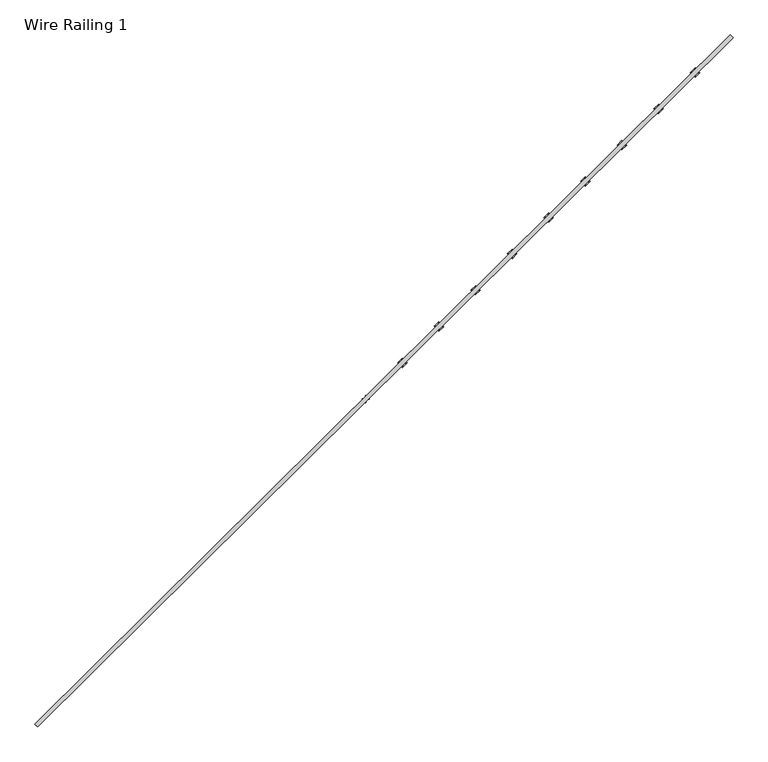
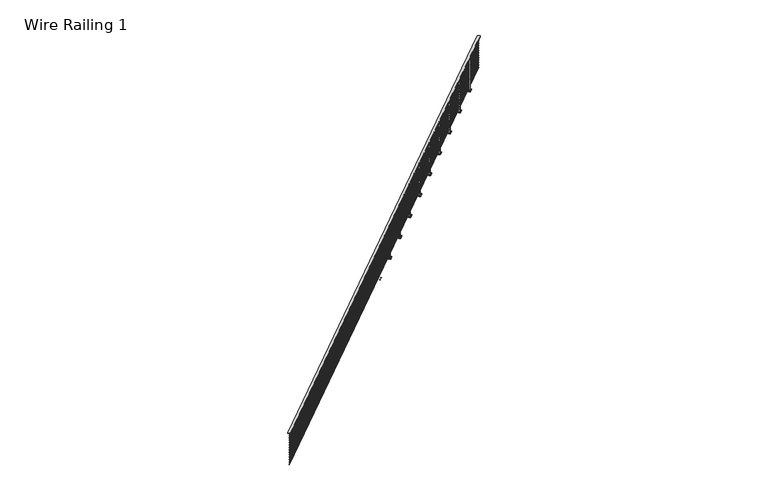
"""IFC4 building model written with IfcOpenShell, lengths in millimetres: railing geometry, Wire Railing 1."""

from ifc_helpers import new_model, si_unit, point, frame, frame_2d, origin, place, context, project, spatial, polyline, circle_curve, trimmed, segment, composite_curve, outline, extrude, source, transform, mapped, element, save


def wire_railing_1_765eeab6(model_context):
    return source(origin(), model_context, "Body", "SweptSolid", [
        extrude(outline(polyline([(32583.8298074, 24310.825617), (32530.1909697, 24364.9487644), (45743.1001377, 37459.6249857), (45796.7389755, 37405.5018383), (32583.8298074, 24310.825617)])), frame((0.0, 0.0, 265004.55), z_axis=(0.0, 0.0, 1.0), x_axis=(1.0, 0.0, 0.0)), (0.0, 0.0, 1.0), 19.05),
        extrude(outline(composite_curve([segment(trimmed(circle_curve(frame_2d((0.0, 2.38125)), 2.38125), [point((-2.38125, 2.38125))], [point((2.38125, 2.38125))], False, "CARTESIAN"), True, "CONTINUOUS"), segment(trimmed(circle_curve(frame_2d((0.0, 2.38125)), 2.38125), [point((2.38125, 2.38125))], [point((-2.38125, 2.38125))], False, "CARTESIAN"), True, "CONTINUOUS")], self_intersect=False)), frame((32557.0103886, 24337.8871907, 264947.4), z_axis=(0.7102775248505508, 0.7039217553763878, 0.0), x_axis=(0.7039217553763878, -0.7102775248505508, 0.0)), (0.0, 0.0, 1.0), 18602.4598918),
        extrude(outline(composite_curve([segment(trimmed(circle_curve(frame_2d((0.0, 2.38125)), 2.38125), [point((-2.38125, 2.38125))], [point((2.38125, 2.38125))], False, "CARTESIAN"), True, "CONTINUOUS"), segment(trimmed(circle_curve(frame_2d((0.0, 2.38125)), 2.38125), [point((2.38125, 2.38125))], [point((-2.38125, 2.38125))], False, "CARTESIAN"), True, "CONTINUOUS")], self_intersect=False)), frame((32557.0103886, 24337.8871907, 264871.2), z_axis=(0.7102775248505508, 0.7039217553763878, 0.0), x_axis=(0.7039217553763878, -0.7102775248505508, 0.0)), (0.0, 0.0, 1.0), 18602.4598918),
        extrude(outline(composite_curve([segment(trimmed(circle_curve(frame_2d((0.0, 2.38125)), 2.38125), [point((-2.38125, 2.38125))], [point((2.38125, 2.38125))], False, "CARTESIAN"), True, "CONTINUOUS"), segment(trimmed(circle_curve(frame_2d((0.0, 2.38125)), 2.38125), [point((2.38125, 2.38125))], [point((-2.38125, 2.38125))], False, "CARTESIAN"), True, "CONTINUOUS")], self_intersect=False)), frame((32557.0103886, 24337.8871907, 264795.0), z_axis=(0.7102775248505508, 0.7039217553763878, 0.0), x_axis=(0.7039217553763878, -0.7102775248505508, 0.0)), (0.0, 0.0, 1.0), 18602.4598918),
        extrude(outline(composite_curve([segment(trimmed(circle_curve(frame_2d((0.0, 2.38125)), 2.38125), [point((-2.38125, 2.38125))], [point((2.38125, 2.38125))], False, "CARTESIAN"), True, "CONTINUOUS"), segment(trimmed(circle_curve(frame_2d((0.0, 2.38125)), 2.38125), [point((2.38125, 2.38125))], [point((-2.38125, 2.38125))], False, "CARTESIAN"), True, "CONTINUOUS")], self_intersect=False)), frame((32557.0103886, 24337.8871907, 264718.8), z_axis=(0.7102775248505508, 0.7039217553763878, 0.0), x_axis=(0.7039217553763878, -0.7102775248505508, 0.0)), (0.0, 0.0, 1.0), 18602.4598918),
        extrude(outline(composite_curve([segment(trimmed(circle_curve(frame_2d((0.0, 2.38125)), 2.38125), [point((-2.38125, 2.38125))], [point((2.38125, 2.38125))], False, "CARTESIAN"), True, "CONTINUOUS"), segment(trimmed(circle_curve(frame_2d((0.0, 2.38125)), 2.38125), [point((2.38125, 2.38125))], [point((-2.38125, 2.38125))], False, "CARTESIAN"), True, "CONTINUOUS")], self_intersect=False)), frame((32557.0103886, 24337.8871907, 264642.6), z_axis=(0.7102775248505508, 0.7039217553763878, 0.0), x_axis=(0.7039217553763878, -0.7102775248505508, 0.0)), (0.0, 0.0, 1.0), 18602.4598918),
        extrude(outline(composite_curve([segment(trimmed(circle_curve(frame_2d((0.0, 2.38125)), 2.38125), [point((-2.38125, 2.38125))], [point((2.38125, 2.38125))], False, "CARTESIAN"), True, "CONTINUOUS"), segment(trimmed(circle_curve(frame_2d((0.0, 2.38125)), 2.38125), [point((2.38125, 2.38125))], [point((-2.38125, 2.38125))], False, "CARTESIAN"), True, "CONTINUOUS")], self_intersect=False)), frame((32557.0103886, 24337.8871907, 264566.4), z_axis=(0.7102775248505508, 0.7039217553763878, 0.0), x_axis=(0.7039217553763878, -0.7102775248505508, 0.0)), (0.0, 0.0, 1.0), 18602.4598918),
        extrude(outline(composite_curve([segment(trimmed(circle_curve(frame_2d((0.0, 2.38125)), 2.38125), [point((-2.38125, 2.38125))], [point((2.38125, 2.38125))], False, "CARTESIAN"), True, "CONTINUOUS"), segment(trimmed(circle_curve(frame_2d((0.0, 2.38125)), 2.38125), [point((2.38125, 2.38125))], [point((-2.38125, 2.38125))], False, "CARTESIAN"), True, "CONTINUOUS")], self_intersect=False)), frame((32557.0103886, 24337.8871907, 264490.2), z_axis=(0.7102775248505508, 0.7039217553763878, 0.0), x_axis=(0.7039217553763878, -0.7102775248505508, 0.0)), (0.0, 0.0, 1.0), 18602.4598918),
        extrude(outline(composite_curve([segment(trimmed(circle_curve(frame_2d((0.0, 2.38125)), 2.38125), [point((-2.38125, 2.38125))], [point((2.38125, 2.38125))], False, "CARTESIAN"), True, "CONTINUOUS"), segment(trimmed(circle_curve(frame_2d((0.0, 2.38125)), 2.38125), [point((2.38125, 2.38125))], [point((-2.38125, 2.38125))], False, "CARTESIAN"), True, "CONTINUOUS")], self_intersect=False)), frame((32557.0103886, 24337.8871907, 264414.0), z_axis=(0.7102775248505508, 0.7039217553763878, 0.0), x_axis=(0.7039217553763878, -0.7102775248505508, 0.0)), (0.0, 0.0, 1.0), 18602.4598918),
        extrude(outline(composite_curve([segment(trimmed(circle_curve(frame_2d((0.0, 2.38125)), 2.38125), [point((-2.38125, 2.38125))], [point((2.38125, 2.38125))], False, "CARTESIAN"), True, "CONTINUOUS"), segment(trimmed(circle_curve(frame_2d((0.0, 2.38125)), 2.38125), [point((2.38125, 2.38125))], [point((-2.38125, 2.38125))], False, "CARTESIAN"), True, "CONTINUOUS")], self_intersect=False)), frame((32557.0103886, 24337.8871907, 264337.8), z_axis=(0.7102775248505508, 0.7039217553763878, 0.0), x_axis=(0.7039217553763878, -0.7102775248505508, 0.0)), (0.0, 0.0, 1.0), 18602.4598918),
        extrude(outline(composite_curve([segment(trimmed(circle_curve(frame_2d((0.0, 2.38125)), 2.38125), [point((-2.38125, 2.38125))], [point((2.38125, 2.38125))], False, "CARTESIAN"), True, "CONTINUOUS"), segment(trimmed(circle_curve(frame_2d((0.0, 2.38125)), 2.38125), [point((2.38125, 2.38125))], [point((-2.38125, 2.38125))], False, "CARTESIAN"), True, "CONTINUOUS")], self_intersect=False)), frame((32557.0103886, 24337.8871907, 264261.6), z_axis=(0.7102775248505508, 0.7039217553763878, 0.0), x_axis=(0.7039217553763878, -0.7102775248505508, 0.0)), (0.0, 0.0, 1.0), 18602.4598918),
        extrude(outline(composite_curve([segment(trimmed(circle_curve(frame_2d((0.0, 2.38125)), 2.38125), [point((-2.38125, 2.38125))], [point((2.38125, 2.38125))], False, "CARTESIAN"), True, "CONTINUOUS"), segment(trimmed(circle_curve(frame_2d((0.0, 2.38125)), 2.38125), [point((2.38125, 2.38125))], [point((-2.38125, 2.38125))], False, "CARTESIAN"), True, "CONTINUOUS")], self_intersect=False)), frame((32557.0103886, 24337.8871907, 264185.4), z_axis=(0.7102775248505508, 0.7039217553763878, 0.0), x_axis=(0.7039217553763878, -0.7102775248505508, 0.0)), (0.0, 0.0, 1.0), 18602.4598918),
        extrude(outline(composite_curve([segment(trimmed(circle_curve(frame_2d((0.0, 2.38125)), 2.38125), [point((-2.38125, 2.38125))], [point((2.38125, 2.38125))], False, "CARTESIAN"), True, "CONTINUOUS"), segment(trimmed(circle_curve(frame_2d((0.0, 2.38125)), 2.38125), [point((2.38125, 2.38125))], [point((-2.38125, 2.38125))], False, "CARTESIAN"), True, "CONTINUOUS")], self_intersect=False)), frame((32557.0103886, 24337.8871907, 264109.2), z_axis=(0.7102775248505508, 0.7039217553763878, 0.0), x_axis=(0.7039217553763878, -0.7102775248505508, 0.0)), (0.0, 0.0, 1.0), 18602.4598918),
        extrude(outline(composite_curve([segment(trimmed(circle_curve(frame_2d((0.0, 2.38125)), 2.38125), [point((-2.38125, 2.38125))], [point((2.38125, 2.38125))], False, "CARTESIAN"), True, "CONTINUOUS"), segment(trimmed(circle_curve(frame_2d((0.0, 2.38125)), 2.38125), [point((2.38125, 2.38125))], [point((-2.38125, 2.38125))], False, "CARTESIAN"), True, "CONTINUOUS")], self_intersect=False)), frame((32557.0103886, 24337.8871907, 264033.0), z_axis=(0.7102775248505508, 0.7039217553763878, 0.0), x_axis=(0.7039217553763878, -0.7102775248505508, 0.0)), (0.0, 0.0, 1.0), 18602.4598918),
        extrude(outline(composite_curve([segment(trimmed(circle_curve(frame_2d((45074.2207706, 36680.5087687)), 6.35), [point((45078.6906738, 36675.9985064))], [point((45069.7508675, 36685.019031))], False, "CARTESIAN"), True, "CONTINUOUS"), segment(trimmed(circle_curve(frame_2d((45074.2207706, 36680.5087687)), 6.35), [point((45069.7508675, 36685.019031))], [point((45078.6906738, 36675.9985064))], False, "CARTESIAN"), True, "CONTINUOUS")], self_intersect=False)), frame((0.0, 0.0, 263956.8), z_axis=(0.0, 0.0, 1.0), x_axis=(1.0, 0.0, 0.0)), (0.0, 0.0, 1.0), 12.7),
        extrude(outline(composite_curve([segment(trimmed(circle_curve(frame_2d((45011.6421266, 36743.6524406)), 6.35), [point((45016.1120297, 36739.1421784))], [point((45007.1722234, 36748.1627029))], False, "CARTESIAN"), True, "CONTINUOUS"), segment(trimmed(circle_curve(frame_2d((45011.6421266, 36743.6524406)), 6.35), [point((45007.1722234, 36748.1627029))], [point((45016.1120297, 36739.1421784))], False, "CARTESIAN"), True, "CONTINUOUS")], self_intersect=False)), frame((0.0, 0.0, 263956.8), z_axis=(0.0, 0.0, 1.0), x_axis=(1.0, 0.0, 0.0)), (0.0, 0.0, 1.0), 12.7),
        extrude(outline(composite_curve([segment(trimmed(circle_curve(frame_2d((45137.3644426, 36743.0874127)), 6.35), [point((45141.8343458, 36738.5771505))], [point((45132.8945395, 36747.597675))], False, "CARTESIAN"), True, "CONTINUOUS"), segment(trimmed(circle_curve(frame_2d((45137.3644426, 36743.0874127)), 6.35), [point((45132.8945395, 36747.597675))], [point((45141.8343458, 36738.5771505))], False, "CARTESIAN"), True, "CONTINUOUS")], self_intersect=False)), frame((0.0, 0.0, 263956.8), z_axis=(0.0, 0.0, 1.0), x_axis=(1.0, 0.0, 0.0)), (0.0, 0.0, 1.0), 12.7),
        extrude(outline(composite_curve([segment(trimmed(circle_curve(frame_2d((45074.7857986, 36806.2310847)), 6.35), [point((45079.2557017, 36801.7208224))], [point((45070.3158954, 36810.741347))], False, "CARTESIAN"), True, "CONTINUOUS"), segment(trimmed(circle_curve(frame_2d((45074.7857986, 36806.2310847)), 6.35), [point((45070.3158954, 36810.741347))], [point((45079.2557017, 36801.7208224))], False, "CARTESIAN"), True, "CONTINUOUS")], self_intersect=False)), frame((0.0, 0.0, 263956.8), z_axis=(0.0, 0.0, 1.0), x_axis=(1.0, 0.0, 0.0)), (0.0, 0.0, 1.0), 12.7),
        extrude(outline(polyline([(44984.7016303, 36743.7735181), (45074.906876, 36833.171581), (45164.3049389, 36742.9663353), (45074.0996932, 36653.5682724), (44984.7016303, 36743.7735181)])), frame((0.0, 0.0, 263956.8), z_axis=(0.0, 0.0, 1.0), x_axis=(1.0, 0.0, 0.0)), (0.0, 0.0, 1.0), 6.35),
        extrude(outline(polyline([(45031.8474988, 36743.5616326), (45074.6949905, 36786.0257125), (45117.1590704, 36743.1782208), (45074.3115787, 36700.7141409), (45031.8474988, 36743.5616326)]), holes=[polyline([(45040.8276642, 36743.5212735), (45074.3519378, 36709.6943063), (45108.178905, 36743.2185799), (45074.6546314, 36777.0455471), (45040.8276642, 36743.5212735)])]), frame((0.0, 0.0, 263956.8), z_axis=(0.0, 0.0, 1.0), x_axis=(1.0, 0.0, 0.0)), (0.0, 0.0, 1.0), 1047.75),
        extrude(outline(composite_curve([segment(trimmed(circle_curve(frame_2d((44378.8044986, 35991.3152834)), 6.35), [point((44383.2744018, 35986.8050211))], [point((44374.3345955, 35995.8255456))], False, "CARTESIAN"), True, "CONTINUOUS"), segment(trimmed(circle_curve(frame_2d((44378.8044986, 35991.3152834)), 6.35), [point((44374.3345955, 35995.8255456))], [point((44383.2744018, 35986.8050211))], False, "CARTESIAN"), True, "CONTINUOUS")], self_intersect=False)), frame((0.0, 0.0, 263956.8), z_axis=(0.0, 0.0, 1.0), x_axis=(1.0, 0.0, 0.0)), (0.0, 0.0, 1.0), 12.7),
        extrude(outline(composite_curve([segment(trimmed(circle_curve(frame_2d((44316.2258546, 36054.4589553)), 6.35), [point((44320.6957577, 36049.948693))], [point((44311.7559514, 36058.9692176))], False, "CARTESIAN"), True, "CONTINUOUS"), segment(trimmed(circle_curve(frame_2d((44316.2258546, 36054.4589553)), 6.35), [point((44311.7559514, 36058.9692176))], [point((44320.6957577, 36049.948693))], False, "CARTESIAN"), True, "CONTINUOUS")], self_intersect=False)), frame((0.0, 0.0, 263956.8), z_axis=(0.0, 0.0, 1.0), x_axis=(1.0, 0.0, 0.0)), (0.0, 0.0, 1.0), 12.7),
        extrude(outline(composite_curve([segment(trimmed(circle_curve(frame_2d((44441.9481706, 36053.8939274)), 6.35), [point((44446.4180738, 36049.3836651))], [point((44437.4782675, 36058.4041897))], False, "CARTESIAN"), True, "CONTINUOUS"), segment(trimmed(circle_curve(frame_2d((44441.9481706, 36053.8939274)), 6.35), [point((44437.4782675, 36058.4041897))], [point((44446.4180738, 36049.3836651))], False, "CARTESIAN"), True, "CONTINUOUS")], self_intersect=False)), frame((0.0, 0.0, 263956.8), z_axis=(0.0, 0.0, 1.0), x_axis=(1.0, 0.0, 0.0)), (0.0, 0.0, 1.0), 12.7),
        extrude(outline(composite_curve([segment(trimmed(circle_curve(frame_2d((44379.3695266, 36117.0375994)), 6.35), [point((44383.8394297, 36112.5273371))], [point((44374.8996234, 36121.5478616))], False, "CARTESIAN"), True, "CONTINUOUS"), segment(trimmed(circle_curve(frame_2d((44379.3695266, 36117.0375994)), 6.35), [point((44374.8996234, 36121.5478616))], [point((44383.8394297, 36112.5273371))], False, "CARTESIAN"), True, "CONTINUOUS")], self_intersect=False)), frame((0.0, 0.0, 263956.8), z_axis=(0.0, 0.0, 1.0), x_axis=(1.0, 0.0, 0.0)), (0.0, 0.0, 1.0), 12.7),
        extrude(outline(polyline([(44289.2853583, 36054.5800327), (44379.490604, 36143.9780957), (44468.8886669, 36053.77285), (44378.6834212, 35964.3747871), (44289.2853583, 36054.5800327)])), frame((0.0, 0.0, 263956.8), z_axis=(0.0, 0.0, 1.0), x_axis=(1.0, 0.0, 0.0)), (0.0, 0.0, 1.0), 6.35),
        extrude(outline(polyline([(44336.4312268, 36054.3681473), (44379.2787185, 36096.8322271), (44421.7427984, 36053.9847355), (44378.8953067, 36011.5206556), (44336.4312268, 36054.3681473)]), holes=[polyline([(44345.4113922, 36054.3277881), (44378.9356658, 36020.500821), (44412.762633, 36054.0250946), (44379.2383594, 36087.8520617), (44345.4113922, 36054.3277881)])]), frame((0.0, 0.0, 263956.8), z_axis=(0.0, 0.0, 1.0), x_axis=(1.0, 0.0, 0.0)), (0.0, 0.0, 1.0), 1047.75),
        extrude(outline(composite_curve([segment(trimmed(circle_curve(frame_2d((43683.3882266, 35302.121798)), 6.35), [point((43687.8581298, 35297.6115357))], [point((43678.9183235, 35306.6320603))], False, "CARTESIAN"), True, "CONTINUOUS"), segment(trimmed(circle_curve(frame_2d((43683.3882266, 35302.121798)), 6.35), [point((43678.9183235, 35306.6320603))], [point((43687.8581298, 35297.6115357))], False, "CARTESIAN"), True, "CONTINUOUS")], self_intersect=False)), frame((0.0, 0.0, 263956.8), z_axis=(0.0, 0.0, 1.0), x_axis=(1.0, 0.0, 0.0)), (0.0, 0.0, 1.0), 12.7),
        extrude(outline(composite_curve([segment(trimmed(circle_curve(frame_2d((43620.8095826, 35365.26547)), 6.35), [point((43625.2794857, 35360.7552077))], [point((43616.3396794, 35369.7757323))], False, "CARTESIAN"), True, "CONTINUOUS"), segment(trimmed(circle_curve(frame_2d((43620.8095826, 35365.26547)), 6.35), [point((43616.3396794, 35369.7757323))], [point((43625.2794857, 35360.7552077))], False, "CARTESIAN"), True, "CONTINUOUS")], self_intersect=False)), frame((0.0, 0.0, 263956.8), z_axis=(0.0, 0.0, 1.0), x_axis=(1.0, 0.0, 0.0)), (0.0, 0.0, 1.0), 12.7),
        extrude(outline(composite_curve([segment(trimmed(circle_curve(frame_2d((43746.5318986, 35364.7004421)), 6.35), [point((43751.0018017, 35360.1901798))], [point((43742.0619955, 35369.2107044))], False, "CARTESIAN"), True, "CONTINUOUS"), segment(trimmed(circle_curve(frame_2d((43746.5318986, 35364.7004421)), 6.35), [point((43742.0619955, 35369.2107044))], [point((43751.0018017, 35360.1901798))], False, "CARTESIAN"), True, "CONTINUOUS")], self_intersect=False)), frame((0.0, 0.0, 263956.8), z_axis=(0.0, 0.0, 1.0), x_axis=(1.0, 0.0, 0.0)), (0.0, 0.0, 1.0), 12.7),
        extrude(outline(composite_curve([segment(trimmed(circle_curve(frame_2d((43683.9532545, 35427.844114)), 6.35), [point((43688.4231577, 35423.3338517))], [point((43679.4833514, 35432.3543763))], False, "CARTESIAN"), True, "CONTINUOUS"), segment(trimmed(circle_curve(frame_2d((43683.9532545, 35427.844114)), 6.35), [point((43679.4833514, 35432.3543763))], [point((43688.4231577, 35423.3338517))], False, "CARTESIAN"), True, "CONTINUOUS")], self_intersect=False)), frame((0.0, 0.0, 263956.8), z_axis=(0.0, 0.0, 1.0), x_axis=(1.0, 0.0, 0.0)), (0.0, 0.0, 1.0), 12.7),
        extrude(outline(polyline([(43593.8690863, 35365.3865474), (43684.074332, 35454.7846103), (43773.4723949, 35364.5793647), (43683.2671492, 35275.1813017), (43593.8690863, 35365.3865474)])), frame((0.0, 0.0, 263956.8), z_axis=(0.0, 0.0, 1.0), x_axis=(1.0, 0.0, 0.0)), (0.0, 0.0, 1.0), 6.35),
        extrude(outline(polyline([(43641.0149548, 35365.1746619), (43683.8624465, 35407.6387418), (43726.3265264, 35364.7912501), (43683.4790347, 35322.3271702), (43641.0149548, 35365.1746619)]), holes=[polyline([(43649.9951202, 35365.1343028), (43683.5193938, 35331.3073357), (43717.346361, 35364.8316093), (43683.8220874, 35398.6585764), (43649.9951202, 35365.1343028)])]), frame((0.0, 0.0, 263956.8), z_axis=(0.0, 0.0, 1.0), x_axis=(1.0, 0.0, 0.0)), (0.0, 0.0, 1.0), 1047.75),
        extrude(outline(composite_curve([segment(trimmed(circle_curve(frame_2d((42987.9719546, 34612.9283127)), 6.35), [point((42992.4418578, 34608.4180504))], [point((42983.5020515, 34617.438575))], False, "CARTESIAN"), True, "CONTINUOUS"), segment(trimmed(circle_curve(frame_2d((42987.9719546, 34612.9283127)), 6.35), [point((42983.5020515, 34617.438575))], [point((42992.4418578, 34608.4180504))], False, "CARTESIAN"), True, "CONTINUOUS")], self_intersect=False)), frame((0.0, 0.0, 263956.8), z_axis=(0.0, 0.0, 1.0), x_axis=(1.0, 0.0, 0.0)), (0.0, 0.0, 1.0), 12.7),
        extrude(outline(composite_curve([segment(trimmed(circle_curve(frame_2d((42925.3933106, 34676.0719846)), 6.35), [point((42929.8632137, 34671.5617224))], [point((42920.9234074, 34680.5822469))], False, "CARTESIAN"), True, "CONTINUOUS"), segment(trimmed(circle_curve(frame_2d((42925.3933106, 34676.0719846)), 6.35), [point((42920.9234074, 34680.5822469))], [point((42929.8632137, 34671.5617224))], False, "CARTESIAN"), True, "CONTINUOUS")], self_intersect=False)), frame((0.0, 0.0, 263956.8), z_axis=(0.0, 0.0, 1.0), x_axis=(1.0, 0.0, 0.0)), (0.0, 0.0, 1.0), 12.7),
        extrude(outline(composite_curve([segment(trimmed(circle_curve(frame_2d((43051.1156266, 34675.5069567)), 6.35), [point((43055.5855297, 34670.9966945))], [point((43046.6457235, 34680.017219))], False, "CARTESIAN"), True, "CONTINUOUS"), segment(trimmed(circle_curve(frame_2d((43051.1156266, 34675.5069567)), 6.35), [point((43046.6457235, 34680.017219))], [point((43055.5855297, 34670.9966945))], False, "CARTESIAN"), True, "CONTINUOUS")], self_intersect=False)), frame((0.0, 0.0, 263956.8), z_axis=(0.0, 0.0, 1.0), x_axis=(1.0, 0.0, 0.0)), (0.0, 0.0, 1.0), 12.7),
        extrude(outline(composite_curve([segment(trimmed(circle_curve(frame_2d((42988.5369825, 34738.6506287)), 6.35), [point((42993.0068857, 34734.1403664))], [point((42984.0670794, 34743.160891))], False, "CARTESIAN"), True, "CONTINUOUS"), segment(trimmed(circle_curve(frame_2d((42988.5369825, 34738.6506287)), 6.35), [point((42984.0670794, 34743.160891))], [point((42993.0068857, 34734.1403664))], False, "CARTESIAN"), True, "CONTINUOUS")], self_intersect=False)), frame((0.0, 0.0, 263956.8), z_axis=(0.0, 0.0, 1.0), x_axis=(1.0, 0.0, 0.0)), (0.0, 0.0, 1.0), 12.7),
        extrude(outline(polyline([(42898.4528143, 34676.1930621), (42988.65806, 34765.591125), (43078.0561229, 34675.3858793), (42987.8508772, 34585.9878164), (42898.4528143, 34676.1930621)])), frame((0.0, 0.0, 263956.8), z_axis=(0.0, 0.0, 1.0), x_axis=(1.0, 0.0, 0.0)), (0.0, 0.0, 1.0), 6.35),
        extrude(outline(polyline([(42945.5986828, 34675.9811766), (42988.4461745, 34718.4452565), (43030.9102544, 34675.5977648), (42988.0627627, 34633.1336849), (42945.5986828, 34675.9811766)]), holes=[polyline([(42954.5788482, 34675.9408175), (42988.1031218, 34642.1138503), (43021.930089, 34675.6381239), (42988.4058154, 34709.4650911), (42954.5788482, 34675.9408175)])]), frame((0.0, 0.0, 263956.8), z_axis=(0.0, 0.0, 1.0), x_axis=(1.0, 0.0, 0.0)), (0.0, 0.0, 1.0), 1047.75),
        extrude(outline(composite_curve([segment(trimmed(circle_curve(frame_2d((42292.5556826, 33923.7348274)), 6.35), [point((42297.0255858, 33919.2245651))], [point((42288.0857795, 33928.2450896))], False, "CARTESIAN"), True, "CONTINUOUS"), segment(trimmed(circle_curve(frame_2d((42292.5556826, 33923.7348274)), 6.35), [point((42288.0857795, 33928.2450896))], [point((42297.0255858, 33919.2245651))], False, "CARTESIAN"), True, "CONTINUOUS")], self_intersect=False)), frame((0.0, 0.0, 263956.8), z_axis=(0.0, 0.0, 1.0), x_axis=(1.0, 0.0, 0.0)), (0.0, 0.0, 1.0), 12.7),
        extrude(outline(composite_curve([segment(trimmed(circle_curve(frame_2d((42229.9770386, 33986.8784993)), 6.35), [point((42234.4469417, 33982.368237))], [point((42225.5071354, 33991.3887616))], False, "CARTESIAN"), True, "CONTINUOUS"), segment(trimmed(circle_curve(frame_2d((42229.9770386, 33986.8784993)), 6.35), [point((42225.5071354, 33991.3887616))], [point((42234.4469417, 33982.368237))], False, "CARTESIAN"), True, "CONTINUOUS")], self_intersect=False)), frame((0.0, 0.0, 263956.8), z_axis=(0.0, 0.0, 1.0), x_axis=(1.0, 0.0, 0.0)), (0.0, 0.0, 1.0), 12.7),
        extrude(outline(composite_curve([segment(trimmed(circle_curve(frame_2d((42355.6993546, 33986.3134714)), 6.35), [point((42360.1692577, 33981.8032091))], [point((42351.2294514, 33990.8237337))], False, "CARTESIAN"), True, "CONTINUOUS"), segment(trimmed(circle_curve(frame_2d((42355.6993546, 33986.3134714)), 6.35), [point((42351.2294514, 33990.8237337))], [point((42360.1692577, 33981.8032091))], False, "CARTESIAN"), True, "CONTINUOUS")], self_intersect=False)), frame((0.0, 0.0, 263956.8), z_axis=(0.0, 0.0, 1.0), x_axis=(1.0, 0.0, 0.0)), (0.0, 0.0, 1.0), 12.7),
        extrude(outline(composite_curve([segment(trimmed(circle_curve(frame_2d((42293.1207105, 34049.4571434)), 6.35), [point((42297.5906137, 34044.9468811))], [point((42288.6508074, 34053.9674056))], False, "CARTESIAN"), True, "CONTINUOUS"), segment(trimmed(circle_curve(frame_2d((42293.1207105, 34049.4571434)), 6.35), [point((42288.6508074, 34053.9674056))], [point((42297.5906137, 34044.9468811))], False, "CARTESIAN"), True, "CONTINUOUS")], self_intersect=False)), frame((0.0, 0.0, 263956.8), z_axis=(0.0, 0.0, 1.0), x_axis=(1.0, 0.0, 0.0)), (0.0, 0.0, 1.0), 12.7),
        extrude(outline(polyline([(42203.0365423, 33986.9995767), (42293.241788, 34076.3976397), (42382.6398509, 33986.192394), (42292.4346052, 33896.7943311), (42203.0365423, 33986.9995767)])), frame((0.0, 0.0, 263956.8), z_axis=(0.0, 0.0, 1.0), x_axis=(1.0, 0.0, 0.0)), (0.0, 0.0, 1.0), 6.35),
        extrude(outline(polyline([(42250.1824108, 33986.7876913), (42293.0299025, 34029.2517711), (42335.4939824, 33986.4042795), (42292.6464907, 33943.9401996), (42250.1824108, 33986.7876913)]), holes=[polyline([(42259.1625762, 33986.7473321), (42292.6868498, 33952.920365), (42326.513817, 33986.4446386), (42292.9895434, 34020.2716057), (42259.1625762, 33986.7473321)])]), frame((0.0, 0.0, 263956.8), z_axis=(0.0, 0.0, 1.0), x_axis=(1.0, 0.0, 0.0)), (0.0, 0.0, 1.0), 1047.75),
        extrude(outline(composite_curve([segment(trimmed(circle_curve(frame_2d((41597.1394106, 33234.541342)), 6.35), [point((41601.6093138, 33230.0310797))], [point((41592.6695075, 33239.0516043))], False, "CARTESIAN"), True, "CONTINUOUS"), segment(trimmed(circle_curve(frame_2d((41597.1394106, 33234.541342)), 6.35), [point((41592.6695075, 33239.0516043))], [point((41601.6093138, 33230.0310797))], False, "CARTESIAN"), True, "CONTINUOUS")], self_intersect=False)), frame((0.0, 0.0, 263956.8), z_axis=(0.0, 0.0, 1.0), x_axis=(1.0, 0.0, 0.0)), (0.0, 0.0, 1.0), 12.7),
        extrude(outline(composite_curve([segment(trimmed(circle_curve(frame_2d((41534.5607666, 33297.685014)), 6.35), [point((41539.0306697, 33293.1747517))], [point((41530.0908634, 33302.1952763))], False, "CARTESIAN"), True, "CONTINUOUS"), segment(trimmed(circle_curve(frame_2d((41534.5607666, 33297.685014)), 6.35), [point((41530.0908634, 33302.1952763))], [point((41539.0306697, 33293.1747517))], False, "CARTESIAN"), True, "CONTINUOUS")], self_intersect=False)), frame((0.0, 0.0, 263956.8), z_axis=(0.0, 0.0, 1.0), x_axis=(1.0, 0.0, 0.0)), (0.0, 0.0, 1.0), 12.7),
        extrude(outline(composite_curve([segment(trimmed(circle_curve(frame_2d((41660.2830826, 33297.1199861)), 6.35), [point((41664.7529857, 33292.6097238))], [point((41655.8131794, 33301.6302484))], False, "CARTESIAN"), True, "CONTINUOUS"), segment(trimmed(circle_curve(frame_2d((41660.2830826, 33297.1199861)), 6.35), [point((41655.8131794, 33301.6302484))], [point((41664.7529857, 33292.6097238))], False, "CARTESIAN"), True, "CONTINUOUS")], self_intersect=False)), frame((0.0, 0.0, 263956.8), z_axis=(0.0, 0.0, 1.0), x_axis=(1.0, 0.0, 0.0)), (0.0, 0.0, 1.0), 12.7),
        extrude(outline(composite_curve([segment(trimmed(circle_curve(frame_2d((41597.7044385, 33360.263658)), 6.35), [point((41602.1743417, 33355.7533957))], [point((41593.2345354, 33364.7739203))], False, "CARTESIAN"), True, "CONTINUOUS"), segment(trimmed(circle_curve(frame_2d((41597.7044385, 33360.263658)), 6.35), [point((41593.2345354, 33364.7739203))], [point((41602.1743417, 33355.7533957))], False, "CARTESIAN"), True, "CONTINUOUS")], self_intersect=False)), frame((0.0, 0.0, 263956.8), z_axis=(0.0, 0.0, 1.0), x_axis=(1.0, 0.0, 0.0)), (0.0, 0.0, 1.0), 12.7),
        extrude(outline(polyline([(41507.6202703, 33297.8060914), (41597.8255159, 33387.2041543), (41687.2235789, 33296.9989087), (41597.0183332, 33207.6008457), (41507.6202703, 33297.8060914)])), frame((0.0, 0.0, 263956.8), z_axis=(0.0, 0.0, 1.0), x_axis=(1.0, 0.0, 0.0)), (0.0, 0.0, 1.0), 6.35),
        extrude(outline(polyline([(41554.7661388, 33297.5942059), (41597.6136305, 33340.0582858), (41640.0777104, 33297.2107941), (41597.2302187, 33254.7467142), (41554.7661388, 33297.5942059)]), holes=[polyline([(41563.7463042, 33297.5538468), (41597.2705778, 33263.7268797), (41631.0975449, 33297.2511533), (41597.5732713, 33331.0781204), (41563.7463042, 33297.5538468)])]), frame((0.0, 0.0, 263956.8), z_axis=(0.0, 0.0, 1.0), x_axis=(1.0, 0.0, 0.0)), (0.0, 0.0, 1.0), 1047.75),
        extrude(outline(composite_curve([segment(trimmed(circle_curve(frame_2d((40901.7231386, 32545.3478567)), 6.35), [point((40906.1930418, 32540.8375944))], [point((40897.2532355, 32549.858119))], False, "CARTESIAN"), True, "CONTINUOUS"), segment(trimmed(circle_curve(frame_2d((40901.7231386, 32545.3478567)), 6.35), [point((40897.2532355, 32549.858119))], [point((40906.1930418, 32540.8375944))], False, "CARTESIAN"), True, "CONTINUOUS")], self_intersect=False)), frame((0.0, 0.0, 263956.8), z_axis=(0.0, 0.0, 1.0), x_axis=(1.0, 0.0, 0.0)), (0.0, 0.0, 1.0), 12.7),
        extrude(outline(composite_curve([segment(trimmed(circle_curve(frame_2d((40839.1444946, 32608.4915286)), 6.35), [point((40843.6143977, 32603.9812664))], [point((40834.6745914, 32613.0017909))], False, "CARTESIAN"), True, "CONTINUOUS"), segment(trimmed(circle_curve(frame_2d((40839.1444946, 32608.4915286)), 6.35), [point((40834.6745914, 32613.0017909))], [point((40843.6143977, 32603.9812664))], False, "CARTESIAN"), True, "CONTINUOUS")], self_intersect=False)), frame((0.0, 0.0, 263956.8), z_axis=(0.0, 0.0, 1.0), x_axis=(1.0, 0.0, 0.0)), (0.0, 0.0, 1.0), 12.7),
        extrude(outline(composite_curve([segment(trimmed(circle_curve(frame_2d((40964.8668106, 32607.9265007)), 6.35), [point((40969.3367137, 32603.4162385))], [point((40960.3969074, 32612.436763))], False, "CARTESIAN"), True, "CONTINUOUS"), segment(trimmed(circle_curve(frame_2d((40964.8668106, 32607.9265007)), 6.35), [point((40960.3969074, 32612.436763))], [point((40969.3367137, 32603.4162385))], False, "CARTESIAN"), True, "CONTINUOUS")], self_intersect=False)), frame((0.0, 0.0, 263956.8), z_axis=(0.0, 0.0, 1.0), x_axis=(1.0, 0.0, 0.0)), (0.0, 0.0, 1.0), 12.7),
        extrude(outline(composite_curve([segment(trimmed(circle_curve(frame_2d((40902.2881665, 32671.0701727)), 6.35), [point((40906.7580697, 32666.5599104))], [point((40897.8182634, 32675.580435))], False, "CARTESIAN"), True, "CONTINUOUS"), segment(trimmed(circle_curve(frame_2d((40902.2881665, 32671.0701727)), 6.35), [point((40897.8182634, 32675.580435))], [point((40906.7580697, 32666.5599104))], False, "CARTESIAN"), True, "CONTINUOUS")], self_intersect=False)), frame((0.0, 0.0, 263956.8), z_axis=(0.0, 0.0, 1.0), x_axis=(1.0, 0.0, 0.0)), (0.0, 0.0, 1.0), 12.7),
        extrude(outline(polyline([(40812.2039983, 32608.6126061), (40902.4092439, 32698.010669), (40991.8073069, 32607.8054233), (40901.6020612, 32518.4073604), (40812.2039983, 32608.6126061)])), frame((0.0, 0.0, 263956.8), z_axis=(0.0, 0.0, 1.0), x_axis=(1.0, 0.0, 0.0)), (0.0, 0.0, 1.0), 6.35),
        extrude(outline(polyline([(40859.3498668, 32608.4007206), (40902.1973585, 32650.8648005), (40944.6614384, 32608.0173088), (40901.8139467, 32565.5532289), (40859.3498668, 32608.4007206)]), holes=[polyline([(40868.3300322, 32608.3603615), (40901.8543058, 32574.5333943), (40935.6812729, 32608.0576679), (40902.1569993, 32641.8846351), (40868.3300322, 32608.3603615)])]), frame((0.0, 0.0, 263956.8), z_axis=(0.0, 0.0, 1.0), x_axis=(1.0, 0.0, 0.0)), (0.0, 0.0, 1.0), 1047.75),
        extrude(outline(composite_curve([segment(trimmed(circle_curve(frame_2d((40206.3068666, 31856.1543714)), 6.35), [point((40210.7767698, 31851.6441091))], [point((40201.8369635, 31860.6646336))], False, "CARTESIAN"), True, "CONTINUOUS"), segment(trimmed(circle_curve(frame_2d((40206.3068666, 31856.1543714)), 6.35), [point((40201.8369635, 31860.6646336))], [point((40210.7767698, 31851.6441091))], False, "CARTESIAN"), True, "CONTINUOUS")], self_intersect=False)), frame((0.0, 0.0, 263956.8), z_axis=(0.0, 0.0, 1.0), x_axis=(1.0, 0.0, 0.0)), (0.0, 0.0, 1.0), 12.7),
        extrude(outline(composite_curve([segment(trimmed(circle_curve(frame_2d((40143.7282226, 31919.2980433)), 6.35), [point((40148.1981257, 31914.787781))], [point((40139.2583194, 31923.8083056))], False, "CARTESIAN"), True, "CONTINUOUS"), segment(trimmed(circle_curve(frame_2d((40143.7282226, 31919.2980433)), 6.35), [point((40139.2583194, 31923.8083056))], [point((40148.1981257, 31914.787781))], False, "CARTESIAN"), True, "CONTINUOUS")], self_intersect=False)), frame((0.0, 0.0, 263956.8), z_axis=(0.0, 0.0, 1.0), x_axis=(1.0, 0.0, 0.0)), (0.0, 0.0, 1.0), 12.7),
        extrude(outline(composite_curve([segment(trimmed(circle_curve(frame_2d((40269.4505386, 31918.7330154)), 6.35), [point((40273.9204417, 31914.2227531))], [point((40264.9806354, 31923.2432777))], False, "CARTESIAN"), True, "CONTINUOUS"), segment(trimmed(circle_curve(frame_2d((40269.4505386, 31918.7330154)), 6.35), [point((40264.9806354, 31923.2432777))], [point((40273.9204417, 31914.2227531))], False, "CARTESIAN"), True, "CONTINUOUS")], self_intersect=False)), frame((0.0, 0.0, 263956.8), z_axis=(0.0, 0.0, 1.0), x_axis=(1.0, 0.0, 0.0)), (0.0, 0.0, 1.0), 12.7),
        extrude(outline(composite_curve([segment(trimmed(circle_curve(frame_2d((40206.8718945, 31981.8766874)), 6.35), [point((40211.3417977, 31977.3664251))], [point((40202.4019914, 31986.3869496))], False, "CARTESIAN"), True, "CONTINUOUS"), segment(trimmed(circle_curve(frame_2d((40206.8718945, 31981.8766874)), 6.35), [point((40202.4019914, 31986.3869496))], [point((40211.3417977, 31977.3664251))], False, "CARTESIAN"), True, "CONTINUOUS")], self_intersect=False)), frame((0.0, 0.0, 263956.8), z_axis=(0.0, 0.0, 1.0), x_axis=(1.0, 0.0, 0.0)), (0.0, 0.0, 1.0), 12.7),
        extrude(outline(polyline([(40116.7877263, 31919.4191207), (40206.9929719, 32008.8171837), (40296.3910349, 31918.611938), (40206.1857892, 31829.2138751), (40116.7877263, 31919.4191207)])), frame((0.0, 0.0, 263956.8), z_axis=(0.0, 0.0, 1.0), x_axis=(1.0, 0.0, 0.0)), (0.0, 0.0, 1.0), 6.35),
        extrude(outline(polyline([(40163.9335948, 31919.2072353), (40206.7810865, 31961.6713151), (40249.2451664, 31918.8238235), (40206.3976747, 31876.3597436), (40163.9335948, 31919.2072353)]), holes=[polyline([(40172.9137602, 31919.1668761), (40206.4380338, 31885.339909), (40240.2650009, 31918.8641826), (40206.7407273, 31952.6911497), (40172.9137602, 31919.1668761)])]), frame((0.0, 0.0, 263956.8), z_axis=(0.0, 0.0, 1.0), x_axis=(1.0, 0.0, 0.0)), (0.0, 0.0, 1.0), 1047.75),
        extrude(outline(composite_curve([segment(trimmed(circle_curve(frame_2d((39510.8905946, 31166.960886)), 6.35), [point((39515.3604978, 31162.4506237))], [point((39506.4206915, 31171.4711483))], False, "CARTESIAN"), True, "CONTINUOUS"), segment(trimmed(circle_curve(frame_2d((39510.8905946, 31166.960886)), 6.35), [point((39506.4206915, 31171.4711483))], [point((39515.3604978, 31162.4506237))], False, "CARTESIAN"), True, "CONTINUOUS")], self_intersect=False)), frame((0.0, 0.0, 263956.8), z_axis=(0.0, 0.0, 1.0), x_axis=(1.0, 0.0, 0.0)), (0.0, 0.0, 1.0), 12.7),
        extrude(outline(composite_curve([segment(trimmed(circle_curve(frame_2d((39448.3119506, 31230.104558)), 6.35), [point((39452.7818537, 31225.5942957))], [point((39443.8420474, 31234.6148203))], False, "CARTESIAN"), True, "CONTINUOUS"), segment(trimmed(circle_curve(frame_2d((39448.3119506, 31230.104558)), 6.35), [point((39443.8420474, 31234.6148203))], [point((39452.7818537, 31225.5942957))], False, "CARTESIAN"), True, "CONTINUOUS")], self_intersect=False)), frame((0.0, 0.0, 263956.8), z_axis=(0.0, 0.0, 1.0), x_axis=(1.0, 0.0, 0.0)), (0.0, 0.0, 1.0), 12.7),
        extrude(outline(composite_curve([segment(trimmed(circle_curve(frame_2d((39574.0342666, 31229.5395301)), 6.35), [point((39578.5041697, 31225.0292678))], [point((39569.5643634, 31234.0497924))], False, "CARTESIAN"), True, "CONTINUOUS"), segment(trimmed(circle_curve(frame_2d((39574.0342666, 31229.5395301)), 6.35), [point((39569.5643634, 31234.0497924))], [point((39578.5041697, 31225.0292678))], False, "CARTESIAN"), True, "CONTINUOUS")], self_intersect=False)), frame((0.0, 0.0, 263956.8), z_axis=(0.0, 0.0, 1.0), x_axis=(1.0, 0.0, 0.0)), (0.0, 0.0, 1.0), 12.7),
        extrude(outline(composite_curve([segment(trimmed(circle_curve(frame_2d((39511.4556225, 31292.683202)), 6.35), [point((39515.9255257, 31288.1729397))], [point((39506.9857194, 31297.1934643))], False, "CARTESIAN"), True, "CONTINUOUS"), segment(trimmed(circle_curve(frame_2d((39511.4556225, 31292.683202)), 6.35), [point((39506.9857194, 31297.1934643))], [point((39515.9255257, 31288.1729397))], False, "CARTESIAN"), True, "CONTINUOUS")], self_intersect=False)), frame((0.0, 0.0, 263956.8), z_axis=(0.0, 0.0, 1.0), x_axis=(1.0, 0.0, 0.0)), (0.0, 0.0, 1.0), 12.7),
        extrude(outline(polyline([(39421.3714543, 31230.2256354), (39511.5766999, 31319.6236983), (39600.9747629, 31229.4184527), (39510.7695172, 31140.0203897), (39421.3714543, 31230.2256354)])), frame((0.0, 0.0, 263956.8), z_axis=(0.0, 0.0, 1.0), x_axis=(1.0, 0.0, 0.0)), (0.0, 0.0, 1.0), 6.35),
        extrude(outline(polyline([(39468.5173228, 31230.0137499), (39511.3648145, 31272.4778298), (39553.8288944, 31229.6303381), (39510.9814027, 31187.1662582), (39468.5173228, 31230.0137499)]), holes=[polyline([(39477.4974882, 31229.9733908), (39511.0217618, 31196.1464237), (39544.8487289, 31229.6706973), (39511.3244553, 31263.4976644), (39477.4974882, 31229.9733908)])]), frame((0.0, 0.0, 263956.8), z_axis=(0.0, 0.0, 1.0), x_axis=(1.0, 0.0, 0.0)), (0.0, 0.0, 1.0), 1047.75),
        extrude(outline(composite_curve([segment(trimmed(circle_curve(frame_2d((38815.4743226, 30477.7674007)), 6.35), [point((38819.9442258, 30473.2571384))], [point((38811.0044195, 30482.277663))], False, "CARTESIAN"), True, "CONTINUOUS"), segment(trimmed(circle_curve(frame_2d((38815.4743226, 30477.7674007)), 6.35), [point((38811.0044195, 30482.277663))], [point((38819.9442258, 30473.2571384))], False, "CARTESIAN"), True, "CONTINUOUS")], self_intersect=False)), frame((0.0, 0.0, 263956.8), z_axis=(0.0, 0.0, 1.0), x_axis=(1.0, 0.0, 0.0)), (0.0, 0.0, 1.0), 12.7),
        extrude(outline(composite_curve([segment(trimmed(circle_curve(frame_2d((38752.8956786, 30540.9110726)), 6.35), [point((38757.3655817, 30536.4008104))], [point((38748.4257754, 30545.4213349))], False, "CARTESIAN"), True, "CONTINUOUS"), segment(trimmed(circle_curve(frame_2d((38752.8956786, 30540.9110726)), 6.35), [point((38748.4257754, 30545.4213349))], [point((38757.3655817, 30536.4008104))], False, "CARTESIAN"), True, "CONTINUOUS")], self_intersect=False)), frame((0.0, 0.0, 263956.8), z_axis=(0.0, 0.0, 1.0), x_axis=(1.0, 0.0, 0.0)), (0.0, 0.0, 1.0), 12.7),
        extrude(outline(composite_curve([segment(trimmed(circle_curve(frame_2d((38878.6179946, 30540.3460447)), 6.35), [point((38883.0878977, 30535.8357825))], [point((38874.1480914, 30544.856307))], False, "CARTESIAN"), True, "CONTINUOUS"), segment(trimmed(circle_curve(frame_2d((38878.6179946, 30540.3460447)), 6.35), [point((38874.1480914, 30544.856307))], [point((38883.0878977, 30535.8357825))], False, "CARTESIAN"), True, "CONTINUOUS")], self_intersect=False)), frame((0.0, 0.0, 263956.8), z_axis=(0.0, 0.0, 1.0), x_axis=(1.0, 0.0, 0.0)), (0.0, 0.0, 1.0), 12.7),
        extrude(outline(composite_curve([segment(trimmed(circle_curve(frame_2d((38816.0393505, 30603.4897167)), 6.35), [point((38820.5092537, 30598.9794544))], [point((38811.5694474, 30607.999979))], False, "CARTESIAN"), True, "CONTINUOUS"), segment(trimmed(circle_curve(frame_2d((38816.0393505, 30603.4897167)), 6.35), [point((38811.5694474, 30607.999979))], [point((38820.5092537, 30598.9794544))], False, "CARTESIAN"), True, "CONTINUOUS")], self_intersect=False)), frame((0.0, 0.0, 263956.8), z_axis=(0.0, 0.0, 1.0), x_axis=(1.0, 0.0, 0.0)), (0.0, 0.0, 1.0), 12.7),
    ])


if __name__ == "__main__":
    model = new_model("IFC4")
    model_context = context("Model", 3, world=origin())
    ifc_project = project(units=[si_unit("LENGTHUNIT", "METRE", prefix="MILLI")], contexts=[model_context])
    site = spatial("IfcSite", under=ifc_project)
    building = spatial("IfcBuilding", under=site)
    placement = place(None, origin())
    wire_railing_1_shape = wire_railing_1_765eeab6(model_context)
    element("IfcRailing", 1, ObjectType="Wire Railing 1", at=placement, inside=building, context=model_context, shape_type="MappedRepresentation", body=[
        mapped(wire_railing_1_shape, transform((0.0, 0.0, 0.0), x_axis=(1.0, 0.0, 0.0), y_axis=(0.0, 1.0, 0.0), z_axis=(0.0, 0.0, 1.0))),
    ])
    save(model, "model.ifc")

# Revit data of these elements
# Element 1 (IfcRailing, "Wire Railing 1")
#   Materials on its faces: "2 1/2\" X 2 1/2\" ALUM. SQUARE POST (38\" O.C. MAX)", "WIRE RAILING (3\" O.C.)", "ALUM. PLATE TOP RAIL"
# Materials
#   "2 1/2\" X 2 1/2\" ALUM. SQUARE POST (38\" O.C. MAX)": class "Metal", colour RGB 244 244 244, transparency 0, Manufacturer = "Kawneer", URL = "http://www.kawneer.com/kawneer/north_america/en/home.asp", Cost = 0
#   "WIRE RAILING (3\" O.C.)": class "Metal", colour RGB 244 244 244, transparency 0, Manufacturer = "Kawneer", URL = "http://www.kawneer.com/kawneer/north_america/en/home.asp", Cost = 0
#   "ALUM. PLATE TOP RAIL": class "Metal", colour RGB 244 244 244, transparency 0, Manufacturer = "Kawneer", URL = "http://www.kawneer.com/kawneer/north_america/en/home.asp", Cost = 0
